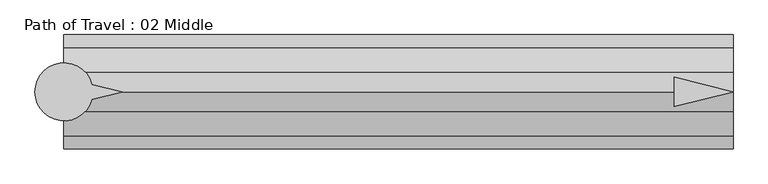
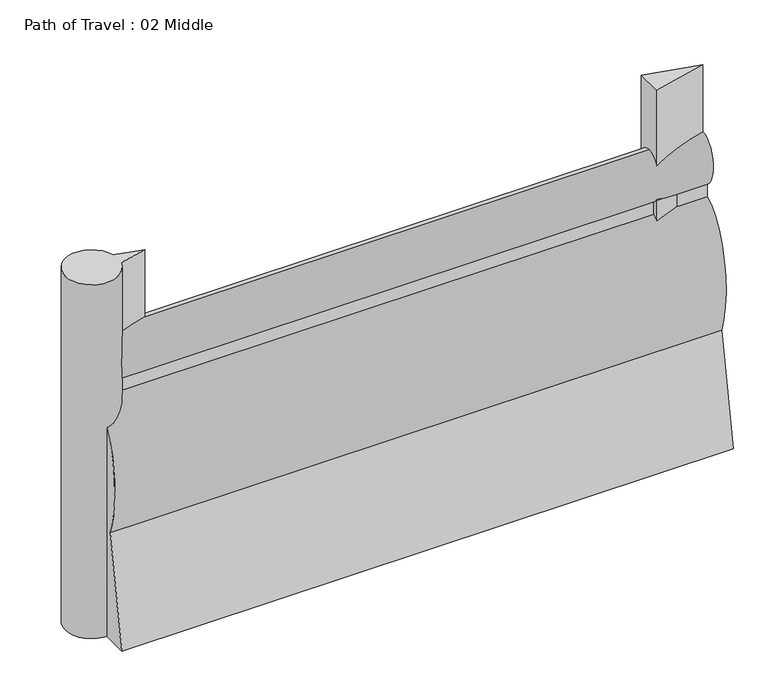
"""IFC4 building model written with IfcOpenShell, lengths in millimetres: proxy geometry, Path of Travel : 02 Middle."""

from ifc_helpers import new_model, si_unit, point, frame, frame_2d, origin, origin_with_axes, place, context, project, spatial, polyline, circle_curve, ellipse_curve, trimmed, segment, composite_curve, outline, extrude, source, transform, mapped, element, save
from ifc_brep_helpers import plane_surface, extruded_surface, advanced_brep


def path_of_travel_02_middle_e76ca7c9(model_context):
    return source(origin(), model_context, "Body", "SolidModel", [
        advanced_brep(
        [(227.5554837, 0.0, 1727.2), (227.5554837, 42.9018657, 1436.6534209), (227.5554837, 42.9018657, 1363.4763406), (227.5554837, 184.1186263, 643.4144547), (227.5554837, 297.5699544, 0.0), (227.5554837, 145.6574193, 0.0), (227.5554837, 0.0, 584.2), (227.5554837, -145.6574193, 0.0), (227.5554837, -297.5699544, 0.0), (227.5554837, -184.1186263, 643.4144547), (227.5554837, -42.9018657, 1363.4763406), (227.5554837, -42.9018657, 1436.6534209), (3707.3554837, 0.0, 1727.2), (3707.3554837, -42.9018657, 1436.6534209), (3707.3554837, -42.9018657, 1363.4763406), (3707.3554837, -184.1186263, 643.4144547), (3707.3554837, -297.5699544, 0.0), (3707.3554837, -145.6574193, 0.0), (3707.3554837, 0.0, 584.2), (3707.3554837, 145.6574193, 0.0), (3707.3554837, 297.5699544, 0.0), (3707.3554837, 184.1186263, 643.4144547), (3707.3554837, 42.9018657, 1363.4763406), (3707.3554837, 42.9018657, 1436.6534209)],
        [
            (0, 1, ellipse_curve(frame((227.5554837, 0.0, 1574.8), z_axis=(-1.0, 0.0, 0.0), x_axis=(0.0, 0.0, 1.0)), 152.4, 101.6)),
            (1, 2),
            (2, 3, ellipse_curve(frame((227.5554837, 0.0, 914.4), z_axis=(-1.0, 0.0, 0.0), x_axis=(0.0, 0.0, -1.0)), 457.2, 228.6)),
            (3, 4),
            (4, 5),
            (5, 6),
            (6, 7),
            (7, 8),
            (8, 9),
            (9, 10, ellipse_curve(frame((227.5554837, 0.0, 914.4), z_axis=(-1.0, 0.0, 0.0), x_axis=(0.0, 0.0, -1.0)), 457.2, 228.6)),
            (10, 11),
            (11, 0, ellipse_curve(frame((227.5554837, 0.0, 1574.8), z_axis=(-1.0, 0.0, 0.0), x_axis=(0.0, 0.0, 1.0)), 152.4, 101.6)),
            (12, 13, ellipse_curve(frame((3707.3554837, 0.0, 1574.8), z_axis=(1.0, 0.0, 0.0), x_axis=(0.0, 0.0, 1.0)), 152.4, 101.6)),
            (13, 14),
            (14, 15, ellipse_curve(frame((3707.3554837, 0.0, 914.4), z_axis=(1.0, 0.0, 0.0), x_axis=(0.0, 0.0, -1.0)), 457.2, 228.6)),
            (15, 16),
            (16, 17),
            (17, 18),
            (18, 19),
            (19, 20),
            (20, 21),
            (21, 22, ellipse_curve(frame((3707.3554837, 0.0, 914.4), z_axis=(1.0, 0.0, 0.0), x_axis=(0.0, 0.0, -1.0)), 457.2, 228.6)),
            (22, 23),
            (23, 12, ellipse_curve(frame((3707.3554837, 0.0, 1574.8), z_axis=(1.0, 0.0, 0.0), x_axis=(0.0, 0.0, 1.0)), 152.4, 101.6)),
            (0, 12),
            (23, 1),
            (22, 2),
            (21, 3),
            (20, 4),
            (19, 5),
            (18, 6),
            (17, 7),
            (16, 8),
            (15, 9),
            (14, 10),
            (13, 11),
        ],
        [
            plane_surface(frame((227.5554837, 0.0, 0.0), z_axis=(-1.0, 0.0, 0.0), x_axis=(0.0, 0.0, 1.0))),
            plane_surface(frame((3707.3554837, 0.0, 0.0), z_axis=(1.0, 0.0, 0.0), x_axis=(0.0, 0.0, 1.0))),
            extruded_surface(trimmed(ellipse_curve(frame((3707.3554837, 0.0, 1574.8), z_axis=(-1.0, 0.0, 0.0), x_axis=(0.0, 0.0, 1.0)), 152.4, 101.6), [point((3707.3554837, 0.0, 1727.2))], [point((3707.3554837, 42.9018657, 1436.6534209))], True, "CARTESIAN"), (-3479.8, 0.0, 0.0), 3479.8),
            plane_surface(frame((227.5554837, 42.9018657, 1436.6534209), z_axis=(0.0, 1.0, 0.0), x_axis=(1.0, 0.0, 0.0))),
            extruded_surface(trimmed(ellipse_curve(frame((3707.3554837, 0.0, 914.4), z_axis=(-1.0, 0.0, 0.0), x_axis=(0.0, 0.0, -1.0)), 457.2, 228.6), [point((3707.3554837, 42.9018657, 1363.4763406))], [point((3707.3554837, 184.1186263, 643.4144547))], True, "CARTESIAN"), (-3479.8, 0.0, 0.0), 3479.8),
            plane_surface(frame((227.5554837, 184.1186263, 643.4144547), z_axis=(0.0, 0.9848077530122078, 0.1736481776669322), x_axis=(1.0, 0.0, 0.0))),
            plane_surface(frame((227.5554837, 297.5699544, 0.0), z_axis=(0.0, 0.0, -1.0), x_axis=(1.0, 0.0, 0.0))),
            plane_surface(frame((227.5554837, 145.6574193, 0.0), z_axis=(0.0, -0.9702957262760199, -0.2419218955995739), x_axis=(1.0, 0.0, 0.0))),
            plane_surface(frame((227.5554837, 0.0, 584.2), z_axis=(0.0, 0.9702957262759961, -0.24192189559966923), x_axis=(1.0, 0.0, 0.0))),
            plane_surface(frame((227.5554837, -145.6574193, 0.0), z_axis=(0.0, 0.0, -1.0), x_axis=(1.0, 0.0, 0.0))),
            plane_surface(frame((227.5554837, -297.5699544, 0.0), z_axis=(0.0, -0.984807753012208, 0.17364817766693066), x_axis=(1.0, 0.0, 0.0))),
            extruded_surface(trimmed(ellipse_curve(frame((3707.3554837, 0.0, 914.4), z_axis=(-1.0, 0.0, 0.0), x_axis=(0.0, 0.0, -1.0)), 457.2, 228.6), [point((3707.3554837, -184.1186263, 643.4144547))], [point((3707.3554837, -42.9018657, 1363.4763406))], True, "CARTESIAN"), (-3479.8, 0.0, 0.0), 3479.8),
            plane_surface(frame((227.5554837, -42.9018657, 1363.4763406), z_axis=(0.0, -1.0, 0.0), x_axis=(1.0, 0.0, 0.0))),
            extruded_surface(trimmed(ellipse_curve(frame((3707.3554837, 0.0, 1574.8), z_axis=(-1.0, 0.0, 0.0), x_axis=(0.0, 0.0, 1.0)), 152.4, 101.6), [point((3707.3554837, -42.9018657, 1436.6534209))], [point((3707.3554837, 0.0, 1727.2))], True, "CARTESIAN"), (-3479.8, 0.0, 0.0), 3479.8),
        ],
        [
            (0, [[1, 2, 3, 4, 5, 6, 7, 8, 9, 10, 11, 12]]),
            (1, [[13, 14, 15, 16, 17, 18, 19, 20, 21, 22, 23, 24]]),
            (2, [[-1, 25, -24, 26]]),
            (3, [[-2, -26, -23, 27]]),
            (4, [[-3, -27, -22, 28]]),
            (5, [[-4, -28, -21, 29]]),
            (6, [[-5, -29, -20, 30]]),
            (7, [[-6, -30, -19, 31]]),
            (8, [[-7, -31, -18, 32]]),
            (9, [[-8, -32, -17, 33]]),
            (10, [[-9, -33, -16, 34]]),
            (11, [[-10, -34, -15, 35]]),
            (12, [[-11, -35, -14, 36]]),
            (13, [[-12, -36, -13, -25]]),
        ],
    ),
        extrude(outline(polyline([(3401.3503371, 76.2006338), (3707.3554837, 0.0), (3401.3503371, -76.2006338), (3401.3503371, 76.2006338)])), origin_with_axes(), (0.0, 0.0, 1.0), 2129.5973753),
        extrude(outline(composite_curve([segment(polyline([(372.7837828, 39.4440225), (531.182385, 0.0), (372.7837828, -39.4440225)]), True, "CONTINUOUS"), segment(trimmed(circle_curve(frame_2d((227.2200886, 0.0)), 150.8131956), [point((372.7837828, -39.4440225))], [point((372.7837828, 39.4440225))], False, "CARTESIAN"), True, "CONTINUOUS")], self_intersect=False)), origin_with_axes(), (0.0, 0.0, 1.0), 2129.5973753),
    ])


if __name__ == "__main__":
    model = new_model("IFC4")
    model_context = context("Model", 3, world=origin())
    ifc_project = project(units=[si_unit("LENGTHUNIT", "METRE", prefix="MILLI")], contexts=[model_context])
    site = spatial("IfcSite", under=ifc_project)
    building = spatial("IfcBuilding", under=site)
    placement = place(None, origin())
    path_of_travel_02_middle_shape = path_of_travel_02_middle_e76ca7c9(model_context)
    element("IfcBuildingElementProxy", 1, Name="Path of Travel : 02 Middle", ObjectType="Path of Travel : 02 Middle", at=placement, inside=building, context=model_context, shape_type="MappedRepresentation", body=[
        mapped(path_of_travel_02_middle_shape, transform((0.0, 0.0, 0.0), x_axis=(1.0, 0.0, 0.0), y_axis=(0.0, 1.0, 0.0), z_axis=(0.0, 0.0, 1.0))),
    ])
    save(model, "model.ifc")

# Revit data of these elements
# Type "Path of Travel : 02 Middle"
#   Path of Egress [instance default] = 4' - 0"
#   built-in parameter 1001306 [instance default] = 4 (stored number, unit not read)
#   Dot at Start = no
#   Arrow in Middle = yes
#   Arrow at End = no
#   Egress Path = none
# Element 1 (IfcBuildingElementProxy, "Path of Travel : 02 Middle")
#   Path of Egress = 11' - 5"
#   built-in parameter 1001306 = 11.4167 (stored number, unit not read)
#   Materials on its faces: "Egress Path Solid", "solid"
# Materials
#   "Egress Path Solid": class "Unassigned", colour RGB 255 128 64, transparency 0.75, Comments = "Rendering appearance not upgraded "
#   "solid": class "Generic", colour RGB 120 120 120, transparency 0, Cost = 0
